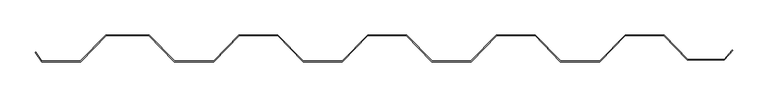
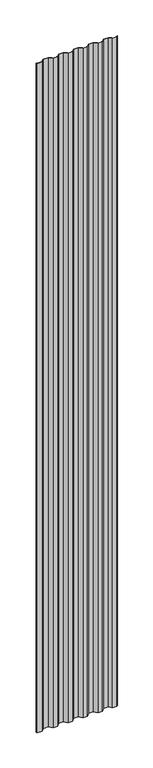
"""IFC4 building model written with IfcOpenShell, lengths in millimetres: proxy geometry, Generic Models 2:Generic Models 2:310765:Generic Models 2:310765 : Generic Models 2:Generic Models 2:310765:84 : Generic Models 2:Generic Models 2:310765:Generic Models 2:310765 : Generic Models 2:Generic Models 2:310765:300385."""

import ifcopenshell
import ifcopenshell.guid

model = None  # the IFC model being written
_history = None  # IfcOwnerHistory: only IFC2X3 demands one
_inside = {}  # id of a spatial element -> (the spatial element, [elements in it])
_under = {}  # id of a project, library or spatial element -> (it, [spatial elements below it])
_declared = {}  # id of a project -> (the project, [libraries it declares])
_typed = {}  # id of a type object -> (the type object, [elements of that type])
_made_of = {}  # id of a material, layer set ... -> (it, [elements and type objects made of it])


def new_model(schema):
    """Start an empty IFC model of exactly this schema.

    Asked for "IFC4X3", IfcOpenShell would pick the latest addendum, in which some entities
    have other attributes; the version numbers below select the first issue.
    IFC2X3 requires an IfcOwnerHistory on every rooted entity: one is made here for all.
    """
    global model, _history
    if schema == "IFC4X3":
        model = ifcopenshell.file(schema_version=(4, 3, 0, 0))
    else:
        model = ifcopenshell.file(schema=schema)
    _inside.clear()
    _under.clear()
    _declared.clear()
    _typed.clear()
    _made_of.clear()
    _history = None
    if model.schema == "IFC2X3":
        org = make("IfcOrganization", Name="unknown")
        user = make(
            "IfcPersonAndOrganization",
            ThePerson=make("IfcPerson", FamilyName="unknown"),
            TheOrganization=org,
        )
        app = make(
            "IfcApplication",
            ApplicationDeveloper=org,
            Version="unknown",
            ApplicationFullName="unknown",
            ApplicationIdentifier="unknown",
        )
        _history = make(
            "IfcOwnerHistory",
            OwningUser=user,
            OwningApplication=app,
            ChangeAction="ADDED",
            CreationDate=0,
        )
    return model


def make(cls, **values):
    """One entity of the class cls with the attributes given. An attribute that is None is left unset."""
    return model.create_entity(
        cls, **{name: value for name, value in values.items() if value is not None}
    )


def rooted(cls, **values):
    """An entity with a GlobalId (a new one), such as an element, a storey or a relation."""
    return make(cls, GlobalId=ifcopenshell.guid.new(), OwnerHistory=_history, **values)


def si_unit(unit_type, name, prefix=None):
    """IfcSIUnit, for example si_unit("LENGTHUNIT", "METRE", prefix="MILLI")."""
    return make("IfcSIUnit", UnitType=unit_type, Prefix=prefix, Name=name)


def assignment(units):
    """IfcUnitAssignment: the units of a project."""
    return None if units is None else make("IfcUnitAssignment", Units=units)


def point(xyz):
    """IfcCartesianPoint."""
    return None if xyz is None else make("IfcCartesianPoint", Coordinates=xyz)


def direction(xyz):
    """IfcDirection."""
    return None if xyz is None else make("IfcDirection", DirectionRatios=xyz)


def frame(location, z_axis=None, x_axis=None):
    """IfcAxis2Placement3D, a coordinate frame: its origin and axes. An axis left out is left unset."""
    return make(
        "IfcAxis2Placement3D",
        Location=point(location),
        Axis=direction(z_axis),
        RefDirection=direction(x_axis),
    )


def origin():
    """The frame at (0, 0, 0) with its axes left unset."""
    return frame((0.0, 0.0, 0.0))


def place(relative_to, where):
    """IfcLocalPlacement: puts the frame where relative to a parent placement (None: the world)."""
    return make(
        "IfcLocalPlacement", PlacementRelTo=relative_to, RelativePlacement=where
    )


def context(
    kind, dimensions, precision=None, world=None, true_north=None, identifier=None
):
    """IfcGeometricRepresentationContext, for example the 3D "Model" context."""
    return make(
        "IfcGeometricRepresentationContext",
        ContextIdentifier=identifier,
        ContextType=kind,
        CoordinateSpaceDimension=dimensions,
        Precision=precision,
        WorldCoordinateSystem=world,
        TrueNorth=true_north,
    )


def project(units=None, contexts=None):
    """IfcProject with its units and contexts."""
    return rooted(
        "IfcProject",
        Name="project",
        RepresentationContexts=contexts,
        UnitsInContext=assignment(units),
    )


def spatial(cls, under=None, at=None, **own):
    """A site, building, storey or space (cls), placed at a placement, below another one or the project."""
    s = rooted(cls, ObjectPlacement=at, **own)
    if under is not None:
        _under.setdefault(under.id(), (under, []))[1].append(s)
    return s


def polyline(points):
    """IfcPolyline through the points."""
    return make("IfcPolyline", Points=[point(p) for p in points])


def outline(outer, holes=None, kind="AREA"):
    """IfcArbitraryClosedProfileDef: a profile drawn as a closed curve; with holes, ...WithVoids."""
    if holes is None:
        return make("IfcArbitraryClosedProfileDef", ProfileType=kind, OuterCurve=outer)
    return make(
        "IfcArbitraryProfileDefWithVoids",
        ProfileType=kind,
        OuterCurve=outer,
        InnerCurves=holes,
    )


def extrude(swept, where, along, depth):
    """IfcExtrudedAreaSolid: the profile swept, set in the frame where, extruded along a direction by depth."""
    return make(
        "IfcExtrudedAreaSolid",
        SweptArea=swept,
        Position=where,
        ExtrudedDirection=direction(along),
        Depth=depth,
    )


def shape(context_of_items, identifier, shape_type, items):
    """IfcShapeRepresentation: the items that make up one representation, for example the "Body"."""
    return make(
        "IfcShapeRepresentation",
        ContextOfItems=context_of_items,
        RepresentationIdentifier=identifier,
        RepresentationType=shape_type,
        Items=items,
    )


def source(mapping_origin, context_of_items, identifier, shape_type, items):
    """IfcRepresentationMap: a shape defined once, which mapped items show again and again."""
    return make(
        "IfcRepresentationMap",
        MappingOrigin=mapping_origin,
        MappedRepresentation=shape(context_of_items, identifier, shape_type, items),
    )


def transform(
    local_origin,
    x_axis=None,
    y_axis=None,
    z_axis=None,
    scale=None,
    scale2=None,
    scale3=None,
    uniform=True,
):
    """IfcCartesianTransformationOperator3D, or its non-uniform kind. x_axis, y_axis, z_axis: its Axis1, 2, 3."""
    if uniform:
        return make(
            "IfcCartesianTransformationOperator3D",
            Axis1=direction(x_axis),
            Axis2=direction(y_axis),
            LocalOrigin=point(local_origin),
            Scale=scale,
            Axis3=direction(z_axis),
        )
    return make(
        "IfcCartesianTransformationOperator3DnonUniform",
        Axis1=direction(x_axis),
        Axis2=direction(y_axis),
        LocalOrigin=point(local_origin),
        Scale=scale,
        Axis3=direction(z_axis),
        Scale2=scale2,
        Scale3=scale3,
    )


def mapped(mapping_source, mapping_target):
    """IfcMappedItem: shows the shape of a source again, moved by a transform."""
    return make(
        "IfcMappedItem", MappingSource=mapping_source, MappingTarget=mapping_target
    )


def made_of(thing, what):
    """Note that an element or type object is made of a material, layer set ...; save() writes the relation."""
    if what is not None:
        _made_of.setdefault(what.id(), (what, []))[1].append(thing)
    return thing


def element(
    cls,
    number,
    at=None,
    inside=None,
    cuts=None,
    type_object=None,
    material=None,
    context=None,
    identifier="Body",
    shape_type=None,
    held_by="IfcProductDefinitionShape",
    body=None,
    shapes=None,
    **own,
):
    """One element of the class cls, such as IfcWall. Its Tag is "e" and its number.

    at: its placement. inside: the storey or other place that contains it. cuts: it is an
    opening in that element (IfcRelVoidsElement). A single representation is given by context,
    identifier, shape_type and body (its items); several are given by shapes. held_by: the class
    of the entity that holds the representations. save() writes the other relations.
    """
    e = rooted(cls, Tag="e%d" % number, ObjectPlacement=at, **own)
    if body is not None:
        shapes = [shape(context, identifier, shape_type, body)]
    if shapes is not None:
        e.Representation = make(held_by, Representations=shapes)
    if inside is not None:
        _inside.setdefault(inside.id(), (inside, []))[1].append(e)
    if cuts is not None:
        rooted(
            "IfcRelVoidsElement", RelatingBuildingElement=cuts, RelatedOpeningElement=e
        )
    if type_object is not None:
        _typed.setdefault(type_object.id(), (type_object, []))[1].append(e)
    return made_of(e, material)


def aggregate(whole, parts):
    """IfcRelAggregates: a whole, such as a stair, and the parts it consists of."""
    return rooted("IfcRelAggregates", RelatingObject=whole, RelatedObjects=parts)


def save(model, path):
    """Write the relations noted so far, then the file.

    IfcRelAggregates (storeys below a building ...), IfcRelContainedInSpatialStructure (elements
    in a storey), IfcRelDefinesByType, IfcRelAssociatesMaterial and IfcRelDeclares: one each for
    every whole, place, type object, material and project.
    """
    for whole, parts in _under.values():
        aggregate(whole, parts)
    for where, things in _inside.values():
        rooted(
            "IfcRelContainedInSpatialStructure",
            RelatedElements=things,
            RelatingStructure=where,
        )
    for kind, things in _typed.values():
        rooted("IfcRelDefinesByType", RelatedObjects=things, RelatingType=kind)
    for what, things in _made_of.values():
        rooted("IfcRelAssociatesMaterial", RelatedObjects=things, RelatingMaterial=what)
    for by, libraries in _declared.values():
        rooted("IfcRelDeclares", RelatingContext=by, RelatedDefinitions=libraries)
    model.write(path)


def generic_models_29386a38(model_context):
    return source(origin(), model_context, "Body", "SweptSolid", [
        extrude(outline(polyline([(593719.8809779, -536567.1923731), (593667.2871722, -536567.1923731), (593633.6551875, -536532.6342858), (593579.1467875, -536532.6342858), (593542.9845958, -536569.9405358), (593486.9373791, -536569.9405358), (593450.7751875, -536532.6342858), (593396.2667875, -536532.6342858), (593360.1045958, -536569.9405358), (593304.0573791, -536569.9405358), (593267.8951875, -536532.6342858), (593213.3867875, -536532.6342858), (593177.2245958, -536569.9405358), (593121.1773791, -536569.9405358), (593085.0151875, -536532.6342858), (593030.5067875, -536532.6342858), (592994.3445958, -536569.9405358), (592938.2973791, -536569.9405358), (592902.1351875, -536532.6342858), (592841.2767875, -536532.6342858), (592805.1145958, -536569.9405358), (592749.8367875, -536569.9405358), (592740.6584173, -536556.8324648), (592741.3086193, -536556.3771885), (592750.2499875, -536569.1467858), (592804.7785503, -536569.1467858), (592840.9407419, -536531.8405358), (592902.471233, -536531.8405358), (592938.6334246, -536569.1467858), (592994.0085503, -536569.1467858), (593030.1707419, -536531.8405358), (593085.351233, -536531.8405358), (593121.5134246, -536569.1467858), (593176.8885503, -536569.1467858), (593213.0507419, -536531.8405358), (593268.231233, -536531.8405358), (593304.3934246, -536569.1467858), (593359.7685503, -536569.1467858), (593395.9307419, -536531.8405358), (593451.111233, -536531.8405358), (593487.2734246, -536569.1467858), (593542.6485503, -536569.1467858), (593578.8107419, -536531.8405358), (593633.9903018, -536531.8405358), (593667.6222866, -536566.3986231), (593719.5286406, -536566.3986231), (593731.1747524, -536553.5223302), (593731.7367242, -536554.084302), (593719.8809779, -536567.1923731)])), frame((0.0, 0.0, -21.9501303), z_axis=(0.0, 0.0, 1.0), x_axis=(1.0, 0.0, 0.0)), (0.0, 0.0, 1.0), 8586.719137),
    ])


if __name__ == "__main__":
    model = new_model("IFC4")
    model_context = context("Model", 3, world=origin())
    ifc_project = project(units=[si_unit("LENGTHUNIT", "METRE", prefix="MILLI")], contexts=[model_context])
    site = spatial("IfcSite", under=ifc_project)
    building = spatial("IfcBuilding", under=site)
    placement = place(None, origin())
    generic_models_shape = generic_models_29386a38(model_context)
    element("IfcBuildingElementProxy", 1, Name="Generic Models 2:Generic Models 2:310765:Generic Models 2:310765 : Generic Models 2:Generic Models 2:310765:84 : Generic Models 2:Generic Models 2:310765:Generic Models 2:310765 : Generic Models 2:Generic Models 2:310765:300385", ObjectType="Generic Models 2:Generic Models 2:310765:Generic Models 2:310765 : Generic Models 2:Generic Models 2:310765:84 : Generic Models 2:Generic Models 2:310765:Generic Models 2:310765 : Generic Models 2:Generic Models 2:310765:300385", at=placement, inside=building, context=model_context, shape_type="MappedRepresentation", body=[
        mapped(generic_models_shape, transform((0.0, 0.0, 0.0), x_axis=(1.0, 0.0, 0.0), y_axis=(0.0, 1.0, 0.0), z_axis=(0.0, 0.0, 1.0))),
    ])
    save(model, "model.ifc")

# Revit data of these elements
# Type "Generic Models 2:Generic Models 2:310765:Generic Models 2:310765 : Generic Models 2:Generic Models 2:310765:84 : Generic Models 2:Generic Models 2:310765:Generic Models 2:310765 : Generic Models 2:Generic Models 2:310765:300385"
#   NameOverride = "Generic Models 2:Generic Models 2:310765:Generic Models 2:310765 : Generic Models 2:Generic Models 2:310765:300385"
#   ObjectTypeOverride = "Generic Models 2:310765 : Generic Models 2:Generic Models 2:310765"
#   Reference = "Generic Models 2"
#   Tag = "300385"
# Element 1 (IfcBuildingElementProxy, "Generic Models 2:Generic Models 2:310765:Generic Models 2:310765 : Generic Models 2:Generic Models 2:310765:84 : Generic Models 2:Generic Models 2:310765:Generic Models 2:310765 : Generic Models 2:Generic Models 2:310765:300385")
#   Materials on its faces: "VERTICAL CORRUGATED METAL PANEL - EXPOSED FASTENERS - (MBCI 7.2 PANEL)"
# Materials
#   "VERTICAL CORRUGATED METAL PANEL - EXPOSED FASTENERS - (MBCI 7.2 PANEL)": class "Generic", colour RGB 120 120 120, transparency 0, Cost = 0
